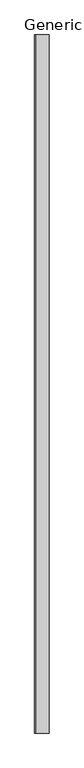
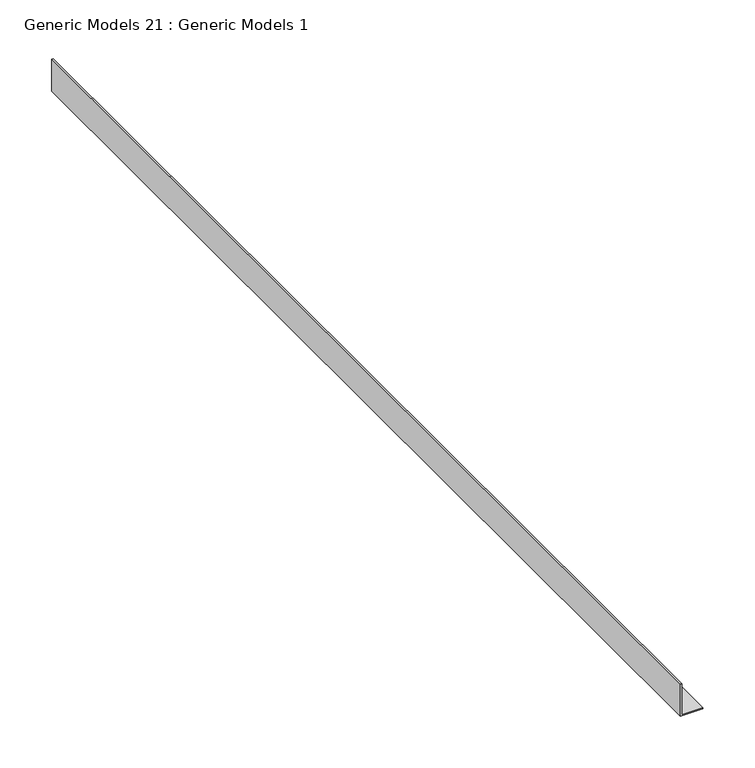
"""IFC4 building model written with IfcOpenShell, lengths in millimetres: proxy geometry, Generic Models 21 : Generic Models 1."""

import ifcopenshell
import ifcopenshell.guid

model = None  # the IFC model being written
_history = None  # IfcOwnerHistory: only IFC2X3 demands one
_inside = {}  # id of a spatial element -> (the spatial element, [elements in it])
_under = {}  # id of a project, library or spatial element -> (it, [spatial elements below it])
_declared = {}  # id of a project -> (the project, [libraries it declares])
_typed = {}  # id of a type object -> (the type object, [elements of that type])
_made_of = {}  # id of a material, layer set ... -> (it, [elements and type objects made of it])


def new_model(schema):
    """Start an empty IFC model of exactly this schema.

    Asked for "IFC4X3", IfcOpenShell would pick the latest addendum, in which some entities
    have other attributes; the version numbers below select the first issue.
    IFC2X3 requires an IfcOwnerHistory on every rooted entity: one is made here for all.
    """
    global model, _history
    if schema == "IFC4X3":
        model = ifcopenshell.file(schema_version=(4, 3, 0, 0))
    else:
        model = ifcopenshell.file(schema=schema)
    _inside.clear()
    _under.clear()
    _declared.clear()
    _typed.clear()
    _made_of.clear()
    _history = None
    if model.schema == "IFC2X3":
        org = make("IfcOrganization", Name="unknown")
        user = make(
            "IfcPersonAndOrganization",
            ThePerson=make("IfcPerson", FamilyName="unknown"),
            TheOrganization=org,
        )
        app = make(
            "IfcApplication",
            ApplicationDeveloper=org,
            Version="unknown",
            ApplicationFullName="unknown",
            ApplicationIdentifier="unknown",
        )
        _history = make(
            "IfcOwnerHistory",
            OwningUser=user,
            OwningApplication=app,
            ChangeAction="ADDED",
            CreationDate=0,
        )
    return model


def make(cls, **values):
    """One entity of the class cls with the attributes given. An attribute that is None is left unset."""
    return model.create_entity(
        cls, **{name: value for name, value in values.items() if value is not None}
    )


def rooted(cls, **values):
    """An entity with a GlobalId (a new one), such as an element, a storey or a relation."""
    return make(cls, GlobalId=ifcopenshell.guid.new(), OwnerHistory=_history, **values)


def si_unit(unit_type, name, prefix=None):
    """IfcSIUnit, for example si_unit("LENGTHUNIT", "METRE", prefix="MILLI")."""
    return make("IfcSIUnit", UnitType=unit_type, Prefix=prefix, Name=name)


def assignment(units):
    """IfcUnitAssignment: the units of a project."""
    return None if units is None else make("IfcUnitAssignment", Units=units)


def point(xyz):
    """IfcCartesianPoint."""
    return None if xyz is None else make("IfcCartesianPoint", Coordinates=xyz)


def direction(xyz):
    """IfcDirection."""
    return None if xyz is None else make("IfcDirection", DirectionRatios=xyz)


def frame(location, z_axis=None, x_axis=None):
    """IfcAxis2Placement3D, a coordinate frame: its origin and axes. An axis left out is left unset."""
    return make(
        "IfcAxis2Placement3D",
        Location=point(location),
        Axis=direction(z_axis),
        RefDirection=direction(x_axis),
    )


def origin():
    """The frame at (0, 0, 0) with its axes left unset."""
    return frame((0.0, 0.0, 0.0))


def place(relative_to, where):
    """IfcLocalPlacement: puts the frame where relative to a parent placement (None: the world)."""
    return make(
        "IfcLocalPlacement", PlacementRelTo=relative_to, RelativePlacement=where
    )


def context(
    kind, dimensions, precision=None, world=None, true_north=None, identifier=None
):
    """IfcGeometricRepresentationContext, for example the 3D "Model" context."""
    return make(
        "IfcGeometricRepresentationContext",
        ContextIdentifier=identifier,
        ContextType=kind,
        CoordinateSpaceDimension=dimensions,
        Precision=precision,
        WorldCoordinateSystem=world,
        TrueNorth=true_north,
    )


def project(units=None, contexts=None):
    """IfcProject with its units and contexts."""
    return rooted(
        "IfcProject",
        Name="project",
        RepresentationContexts=contexts,
        UnitsInContext=assignment(units),
    )


def spatial(cls, under=None, at=None, **own):
    """A site, building, storey or space (cls), placed at a placement, below another one or the project."""
    s = rooted(cls, ObjectPlacement=at, **own)
    if under is not None:
        _under.setdefault(under.id(), (under, []))[1].append(s)
    return s


def polyline(points):
    """IfcPolyline through the points."""
    return make("IfcPolyline", Points=[point(p) for p in points])


def outline(outer, holes=None, kind="AREA"):
    """IfcArbitraryClosedProfileDef: a profile drawn as a closed curve; with holes, ...WithVoids."""
    if holes is None:
        return make("IfcArbitraryClosedProfileDef", ProfileType=kind, OuterCurve=outer)
    return make(
        "IfcArbitraryProfileDefWithVoids",
        ProfileType=kind,
        OuterCurve=outer,
        InnerCurves=holes,
    )


def extrude(swept, where, along, depth):
    """IfcExtrudedAreaSolid: the profile swept, set in the frame where, extruded along a direction by depth."""
    return make(
        "IfcExtrudedAreaSolid",
        SweptArea=swept,
        Position=where,
        ExtrudedDirection=direction(along),
        Depth=depth,
    )


def shape(context_of_items, identifier, shape_type, items):
    """IfcShapeRepresentation: the items that make up one representation, for example the "Body"."""
    return make(
        "IfcShapeRepresentation",
        ContextOfItems=context_of_items,
        RepresentationIdentifier=identifier,
        RepresentationType=shape_type,
        Items=items,
    )


def source(mapping_origin, context_of_items, identifier, shape_type, items):
    """IfcRepresentationMap: a shape defined once, which mapped items show again and again."""
    return make(
        "IfcRepresentationMap",
        MappingOrigin=mapping_origin,
        MappedRepresentation=shape(context_of_items, identifier, shape_type, items),
    )


def transform(
    local_origin,
    x_axis=None,
    y_axis=None,
    z_axis=None,
    scale=None,
    scale2=None,
    scale3=None,
    uniform=True,
):
    """IfcCartesianTransformationOperator3D, or its non-uniform kind. x_axis, y_axis, z_axis: its Axis1, 2, 3."""
    if uniform:
        return make(
            "IfcCartesianTransformationOperator3D",
            Axis1=direction(x_axis),
            Axis2=direction(y_axis),
            LocalOrigin=point(local_origin),
            Scale=scale,
            Axis3=direction(z_axis),
        )
    return make(
        "IfcCartesianTransformationOperator3DnonUniform",
        Axis1=direction(x_axis),
        Axis2=direction(y_axis),
        LocalOrigin=point(local_origin),
        Scale=scale,
        Axis3=direction(z_axis),
        Scale2=scale2,
        Scale3=scale3,
    )


def mapped(mapping_source, mapping_target):
    """IfcMappedItem: shows the shape of a source again, moved by a transform."""
    return make(
        "IfcMappedItem", MappingSource=mapping_source, MappingTarget=mapping_target
    )


def made_of(thing, what):
    """Note that an element or type object is made of a material, layer set ...; save() writes the relation."""
    if what is not None:
        _made_of.setdefault(what.id(), (what, []))[1].append(thing)
    return thing


def element(
    cls,
    number,
    at=None,
    inside=None,
    cuts=None,
    type_object=None,
    material=None,
    context=None,
    identifier="Body",
    shape_type=None,
    held_by="IfcProductDefinitionShape",
    body=None,
    shapes=None,
    **own,
):
    """One element of the class cls, such as IfcWall. Its Tag is "e" and its number.

    at: its placement. inside: the storey or other place that contains it. cuts: it is an
    opening in that element (IfcRelVoidsElement). A single representation is given by context,
    identifier, shape_type and body (its items); several are given by shapes. held_by: the class
    of the entity that holds the representations. save() writes the other relations.
    """
    e = rooted(cls, Tag="e%d" % number, ObjectPlacement=at, **own)
    if body is not None:
        shapes = [shape(context, identifier, shape_type, body)]
    if shapes is not None:
        e.Representation = make(held_by, Representations=shapes)
    if inside is not None:
        _inside.setdefault(inside.id(), (inside, []))[1].append(e)
    if cuts is not None:
        rooted(
            "IfcRelVoidsElement", RelatingBuildingElement=cuts, RelatedOpeningElement=e
        )
    if type_object is not None:
        _typed.setdefault(type_object.id(), (type_object, []))[1].append(e)
    return made_of(e, material)


def aggregate(whole, parts):
    """IfcRelAggregates: a whole, such as a stair, and the parts it consists of."""
    return rooted("IfcRelAggregates", RelatingObject=whole, RelatedObjects=parts)


def save(model, path):
    """Write the relations noted so far, then the file.

    IfcRelAggregates (storeys below a building ...), IfcRelContainedInSpatialStructure (elements
    in a storey), IfcRelDefinesByType, IfcRelAssociatesMaterial and IfcRelDeclares: one each for
    every whole, place, type object, material and project.
    """
    for whole, parts in _under.values():
        aggregate(whole, parts)
    for where, things in _inside.values():
        rooted(
            "IfcRelContainedInSpatialStructure",
            RelatedElements=things,
            RelatingStructure=where,
        )
    for kind, things in _typed.values():
        rooted("IfcRelDefinesByType", RelatedObjects=things, RelatingType=kind)
    for what, things in _made_of.values():
        rooted("IfcRelAssociatesMaterial", RelatedObjects=things, RelatingMaterial=what)
    for by, libraries in _declared.values():
        rooted("IfcRelDeclares", RelatingContext=by, RelatedDefinitions=libraries)
    model.write(path)


def generic_models_21_generic_models_1_e8c90d4c(model_context):
    return source(origin(), model_context, "Body", "SweptSolid", [
        extrude(outline(polyline([(2277.1204978, 49799.875), (2239.0204978, 49799.875), (2239.0204978, 49825.275), (2240.6079978, 49825.275), (2240.6079978, 49801.4625), (2277.1204978, 49801.4625), (2277.1204978, 49799.875)])), frame((0.0, 0.0, 0.0), z_axis=(0.0, 1.0, 0.0), x_axis=(0.0, 0.0, 1.0)), (0.0, 0.0, 1.0), 1219.2),
    ])


if __name__ == "__main__":
    model = new_model("IFC4")
    model_context = context("Model", 3, world=origin())
    ifc_project = project(units=[si_unit("LENGTHUNIT", "METRE", prefix="MILLI")], contexts=[model_context])
    site = spatial("IfcSite", under=ifc_project)
    building = spatial("IfcBuilding", under=site)
    placement = place(None, origin())
    generic_models_21_generic_models_1_shape = generic_models_21_generic_models_1_e8c90d4c(model_context)
    element("IfcBuildingElementProxy", 1, Name="Generic Models 21 : Generic Models 1", ObjectType="Generic Models 21 : Generic Models 1", at=placement, inside=building, context=model_context, shape_type="MappedRepresentation", body=[
        mapped(generic_models_21_generic_models_1_shape, transform((0.0, 0.0, 0.0), x_axis=(1.0, 0.0, 0.0), y_axis=(0.0, 1.0, 0.0), z_axis=(0.0, 0.0, 1.0))),
    ])
    save(model, "model.ifc")

# Revit data of these elements
# Element 1 (IfcBuildingElementProxy, "Generic Models 21 : Generic Models 1")
#   Materials on its faces: "CEILING TRACK AS SCHEDULED"
# Materials
#   "CEILING TRACK AS SCHEDULED": class "Unassigned", colour RGB 210 209 208, transparency 0, Keynote = "M05121300.02", Cost = 0
